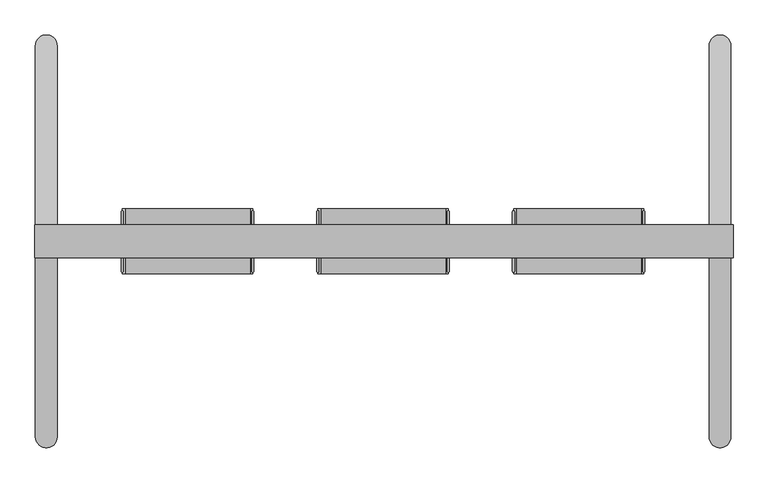
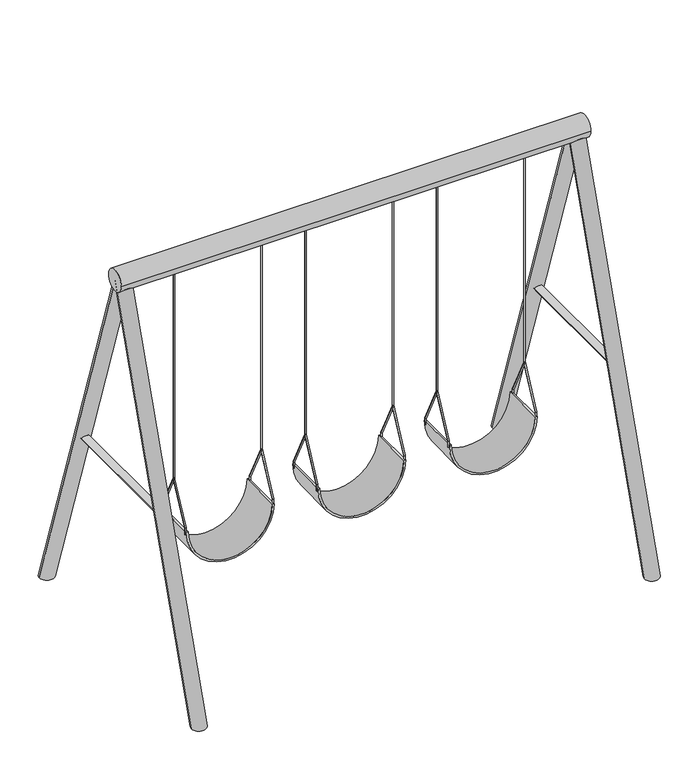
"""IFC4 building model written with IfcOpenShell, lengths in millimetres: geographic element geometry, NLRS_90_SI_WPB_schommel_gen_rsf : schommel drie zittingen."""

from ifc_helpers import new_model, si_unit, point, frame, frame_2d, origin, place, context, project, spatial, polyline, circle_curve, ellipse_curve, trimmed, segment, composite_curve, outline, extrude, source, transform, mapped, element, save
from ifc_brep_helpers import plane_surface, cylinder_surface, extruded_surface, advanced_brep


def geographic_element_11561118(model_context):
    return source(origin(), model_context, "Body", "SolidModel", [
        extrude(outline(composite_curve([segment(trimmed(circle_curve(frame_2d((1554.4555861, -208.1099379)), 4.8239671), [point((1549.631619, -208.1099379))], [point((1559.2795532, -208.1099379))], False, "CARTESIAN"), True, "CONTINUOUS"), segment(trimmed(circle_curve(frame_2d((1554.4555861, -208.1099379)), 4.8239671), [point((1559.2795532, -208.1099379))], [point((1549.631619, -208.1099379))], False, "CARTESIAN"), True, "CONTINUOUS")], self_intersect=False)), frame((0.0, 0.0, 1142.0124483), z_axis=(0.0, 0.0, 1.0), x_axis=(1.0, 0.0, 0.0)), (0.0, 0.0, 1.0), 1601.1875517),
        extrude(outline(composite_curve([segment(trimmed(circle_curve(frame_2d((944.8555861, -208.1099379)), 4.8239671), [point((940.031619, -208.1099379))], [point((949.6795532, -208.1099379))], False, "CARTESIAN"), True, "CONTINUOUS"), segment(trimmed(circle_curve(frame_2d((944.8555861, -208.1099379)), 4.8239671), [point((949.6795532, -208.1099379))], [point((940.031619, -208.1099379))], False, "CARTESIAN"), True, "CONTINUOUS")], self_intersect=False)), frame((0.0, 0.0, 1142.0124483), z_axis=(0.0, 0.0, 1.0), x_axis=(1.0, 0.0, 0.0)), (0.0, 0.0, 1.0), 1601.1875517),
        extrude(outline(composite_curve([segment(trimmed(circle_curve(frame_2d((640.0555861, -208.1099379)), 4.8239671), [point((635.231619, -208.1099379))], [point((644.8795532, -208.1099379))], False, "CARTESIAN"), True, "CONTINUOUS"), segment(trimmed(circle_curve(frame_2d((640.0555861, -208.1099379)), 4.8239671), [point((644.8795532, -208.1099379))], [point((635.231619, -208.1099379))], False, "CARTESIAN"), True, "CONTINUOUS")], self_intersect=False)), frame((0.0, 0.0, 1142.0124483), z_axis=(0.0, 0.0, 1.0), x_axis=(1.0, 0.0, 0.0)), (0.0, 0.0, 1.0), 1601.1875517),
        extrude(outline(composite_curve([segment(trimmed(circle_curve(frame_2d((30.4555861, -208.1099379)), 4.8239671), [point((25.631619, -208.1099379))], [point((35.2795532, -208.1099379))], False, "CARTESIAN"), True, "CONTINUOUS"), segment(trimmed(circle_curve(frame_2d((30.4555861, -208.1099379)), 4.8239671), [point((35.2795532, -208.1099379))], [point((25.631619, -208.1099379))], False, "CARTESIAN"), True, "CONTINUOUS")], self_intersect=False)), frame((0.0, 0.0, 1142.0124483), z_axis=(0.0, 0.0, 1.0), x_axis=(1.0, 0.0, 0.0)), (0.0, 0.0, 1.0), 1601.1875517),
        extrude(outline(composite_curve([segment(trimmed(circle_curve(frame_2d((-274.3444139, -208.1099379)), 4.8239671), [point((-279.168381, -208.1099379))], [point((-269.5204468, -208.1099379))], False, "CARTESIAN"), True, "CONTINUOUS"), segment(trimmed(circle_curve(frame_2d((-274.3444139, -208.1099379)), 4.8239671), [point((-269.5204468, -208.1099379))], [point((-279.168381, -208.1099379))], False, "CARTESIAN"), True, "CONTINUOUS")], self_intersect=False)), frame((0.0, 0.0, 1142.0124483), z_axis=(0.0, 0.0, 1.0), x_axis=(1.0, 0.0, 0.0)), (0.0, 0.0, 1.0), 1601.1875517),
        extrude(outline(composite_curve([segment(trimmed(circle_curve(frame_2d((-884.281587, -208.1099379)), 4.8239671), [point((-889.1055542, -208.1099379))], [point((-879.4576199, -208.1099379))], False, "CARTESIAN"), True, "CONTINUOUS"), segment(trimmed(circle_curve(frame_2d((-884.281587, -208.1099379)), 4.8239671), [point((-879.4576199, -208.1099379))], [point((-889.1055542, -208.1099379))], False, "CARTESIAN"), True, "CONTINUOUS")], self_intersect=False)), frame((0.0, 0.0, 1142.0124483), z_axis=(0.0, 0.0, 1.0), x_axis=(1.0, 0.0, 0.0)), (0.0, 0.0, 1.0), 1601.1875517),
        advanced_brep(
        [(1859.2555861, -1121.8740789, 0.0), (1960.8555861, -1121.8740789, 0.0), (1960.8555861, -207.4740789, 2743.2), (1859.2555861, -207.4740789, 2743.2)],
        [
            (0, 1, circle_curve(frame((1910.0555861, -1121.8740789, 0.0), z_axis=(0.0, 0.0, 1.0), x_axis=(-1.0, 0.0, 0.0)), 50.8)),
            (1, 2),
            (2, 3, circle_curve(frame((1910.0555861, -207.4740789, 2743.2), z_axis=(0.0, 0.0, -1.0), x_axis=(-1.0, 0.0, 0.0)), 50.8)),
            (3, 0),
            (0, 1, circle_curve(frame((1910.0555861, -1121.8740789, 0.0), z_axis=(0.0, 0.0, -1.0), x_axis=(-1.0, 0.0, 0.0)), 50.8)),
            (3, 2, circle_curve(frame((1910.0555861, -207.4740789, 2743.2), z_axis=(0.0, 0.0, -1.0), x_axis=(-1.0, 0.0, 0.0)), 50.8)),
        ],
        [
            extruded_surface(trimmed(circle_curve(frame((1910.0555861, -1121.8740789, 0.0), z_axis=(0.0, 0.0, 1.0), x_axis=(-1.0, 0.0, 0.0)), 50.8), [point((1859.2555861, -1121.8740789, 0.0))], [point((1960.8555861, -1121.8740789, 0.0))], True, "CARTESIAN"), (0.0, 914.4000000000001, 2743.2), 2891.586692457966),
            plane_surface(frame((1910.0555861, -1121.8740789, 0.0), z_axis=(0.0, 0.0, -1.0), x_axis=(0.0, 1.0, 0.0))),
            extruded_surface(trimmed(circle_curve(frame((1910.0555861, -1121.8740789, 0.0), z_axis=(0.0, 0.0, 1.0), x_axis=(-1.0, 0.0, 0.0)), 50.8), [point((1960.8555861, -1121.8740789, 0.0))], [point((1859.2555861, -1121.8740789, 0.0))], True, "CARTESIAN"), (0.0, 914.4000000000001, 2743.2), 2891.586692457966),
            plane_surface(frame((1910.0555861, -207.4740789, 2743.2), z_axis=(0.0, 0.0, 1.0), x_axis=(0.0, 1.0, 0.0))),
        ],
        [
            (0, [[1, 2, 3, 4]]),
            (1, [[-1, 5]]),
            (2, [[-5, -4, 6, -2]]),
            (3, [[-6, -3]]),
        ],
    ),
        advanced_brep(
        [(1859.2555861, 706.9259211, 0.0), (1960.8555861, 706.9259211, 0.0), (1960.8555861, -207.4740789, 2743.2), (1859.2555861, -207.4740789, 2743.2)],
        [
            (0, 1, circle_curve(frame((1910.0555861, 706.9259211, 0.0), z_axis=(0.0, 0.0, 1.0), x_axis=(-1.0, 0.0, 0.0)), 50.8)),
            (1, 2),
            (2, 3, circle_curve(frame((1910.0555861, -207.4740789, 2743.2), z_axis=(0.0, 0.0, -1.0), x_axis=(-1.0, 0.0, 0.0)), 50.8)),
            (3, 0),
            (0, 1, circle_curve(frame((1910.0555861, 706.9259211, 0.0), z_axis=(0.0, 0.0, -1.0), x_axis=(-1.0, 0.0, 0.0)), 50.8)),
            (3, 2, circle_curve(frame((1910.0555861, -207.4740789, 2743.2), z_axis=(0.0, 0.0, -1.0), x_axis=(-1.0, 0.0, 0.0)), 50.8)),
        ],
        [
            extruded_surface(trimmed(circle_curve(frame((1910.0555861, 706.9259211, 0.0), z_axis=(0.0, 0.0, 1.0), x_axis=(-1.0, 0.0, 0.0)), 50.8), [point((1859.2555861, 706.9259211, 0.0))], [point((1960.8555861, 706.9259211, 0.0))], True, "CARTESIAN"), (0.0, -914.4, 2743.2), 2891.586692457966),
            plane_surface(frame((1910.0555861, 706.9259211, 0.0), z_axis=(0.0, 0.0, -1.0), x_axis=(0.0, 1.0, 0.0))),
            extruded_surface(trimmed(circle_curve(frame((1910.0555861, 706.9259211, 0.0), z_axis=(0.0, 0.0, 1.0), x_axis=(-1.0, 0.0, 0.0)), 50.8), [point((1960.8555861, 706.9259211, 0.0))], [point((1859.2555861, 706.9259211, 0.0))], True, "CARTESIAN"), (0.0, -914.4, 2743.2), 2891.586692457966),
            plane_surface(frame((1910.0555861, -207.4740789, 2743.2), z_axis=(0.0, 0.0, 1.0), x_axis=(0.0, 1.0, 0.0))),
        ],
        [
            (0, [[1, 2, 3, 4]]),
            (1, [[-1, 5]]),
            (2, [[-5, -4, 6, -2]]),
            (3, [[-6, -3]]),
        ],
    ),
        advanced_brep(
        [(-1188.7444139, -1121.8740789, 0.0), (-1290.3444139, -1121.8740789, 0.0), (-1290.3444139, -207.4740789, 2743.2), (-1188.7444139, -207.4740789, 2743.2)],
        [
            (0, 1, circle_curve(frame((-1239.5444139, -1121.8740789, 0.0), z_axis=(0.0, 0.0, 1.0), x_axis=(1.0, 0.0, 0.0)), 50.8)),
            (1, 2),
            (2, 3, circle_curve(frame((-1239.5444139, -207.4740789, 2743.2), z_axis=(0.0, 0.0, -1.0), x_axis=(1.0, 0.0, 0.0)), 50.8)),
            (3, 0),
            (0, 1, circle_curve(frame((-1239.5444139, -1121.8740789, 0.0), z_axis=(0.0, 0.0, -1.0), x_axis=(1.0, 0.0, 0.0)), 50.8)),
            (3, 2, circle_curve(frame((-1239.5444139, -207.4740789, 2743.2), z_axis=(0.0, 0.0, -1.0), x_axis=(1.0, 0.0, 0.0)), 50.8)),
        ],
        [
            extruded_surface(trimmed(circle_curve(frame((-1239.5444139, -1121.8740789, 0.0), z_axis=(0.0, 0.0, 1.0), x_axis=(1.0, 0.0, 0.0)), 50.8), [point((-1188.7444139, -1121.8740789, 0.0))], [point((-1290.3444139, -1121.8740789, 0.0))], True, "CARTESIAN"), (0.0, 914.4000000000001, 2743.2), 2891.586692457966),
            plane_surface(frame((-1239.5444139, -1121.8740789, 0.0), z_axis=(0.0, 0.0, -1.0), x_axis=(0.0, -1.0, 0.0))),
            extruded_surface(trimmed(circle_curve(frame((-1239.5444139, -1121.8740789, 0.0), z_axis=(0.0, 0.0, 1.0), x_axis=(1.0, 0.0, 0.0)), 50.8), [point((-1290.3444139, -1121.8740789, 0.0))], [point((-1188.7444139, -1121.8740789, 0.0))], True, "CARTESIAN"), (0.0, 914.4000000000001, 2743.2), 2891.586692457966),
            plane_surface(frame((-1239.5444139, -207.4740789, 2743.2), z_axis=(0.0, 0.0, 1.0), x_axis=(0.0, -1.0, 0.0))),
        ],
        [
            (0, [[1, 2, 3, 4]]),
            (1, [[-1, 5]]),
            (2, [[-5, -4, 6, -2]]),
            (3, [[-6, -3]]),
        ],
    ),
        advanced_brep(
        [(-1188.7444139, 706.9259211, 0.0), (-1290.3444139, 706.9259211, 0.0), (-1290.3444139, -207.4740789, 2743.2), (-1188.7444139, -207.4740789, 2743.2)],
        [
            (0, 1, circle_curve(frame((-1239.5444139, 706.9259211, 0.0), z_axis=(0.0, 0.0, 1.0), x_axis=(1.0, 0.0, 0.0)), 50.8)),
            (1, 2),
            (2, 3, circle_curve(frame((-1239.5444139, -207.4740789, 2743.2), z_axis=(0.0, 0.0, -1.0), x_axis=(1.0, 0.0, 0.0)), 50.8)),
            (3, 0),
            (0, 1, circle_curve(frame((-1239.5444139, 706.9259211, 0.0), z_axis=(0.0, 0.0, -1.0), x_axis=(1.0, 0.0, 0.0)), 50.8)),
            (3, 2, circle_curve(frame((-1239.5444139, -207.4740789, 2743.2), z_axis=(0.0, 0.0, -1.0), x_axis=(1.0, 0.0, 0.0)), 50.8)),
        ],
        [
            extruded_surface(trimmed(circle_curve(frame((-1239.5444139, 706.9259211, 0.0), z_axis=(0.0, 0.0, 1.0), x_axis=(1.0, 0.0, 0.0)), 50.8), [point((-1188.7444139, 706.9259211, 0.0))], [point((-1290.3444139, 706.9259211, 0.0))], True, "CARTESIAN"), (0.0, -914.4, 2743.2), 2891.586692457966),
            plane_surface(frame((-1239.5444139, 706.9259211, 0.0), z_axis=(0.0, 0.0, -1.0), x_axis=(0.0, -1.0, 0.0))),
            extruded_surface(trimmed(circle_curve(frame((-1239.5444139, 706.9259211, 0.0), z_axis=(0.0, 0.0, 1.0), x_axis=(1.0, 0.0, 0.0)), 50.8), [point((-1290.3444139, 706.9259211, 0.0))], [point((-1188.7444139, 706.9259211, 0.0))], True, "CARTESIAN"), (0.0, -914.4, 2743.2), 2891.586692457966),
            plane_surface(frame((-1239.5444139, -207.4740789, 2743.2), z_axis=(0.0, 0.0, 1.0), x_axis=(0.0, -1.0, 0.0))),
        ],
        [
            (0, [[1, 2, 3, 4]]),
            (1, [[-1, 5]]),
            (2, [[-5, -4, 6, -2]]),
            (3, [[-6, -3]]),
        ],
    ),
        extrude(outline(composite_curve([segment(trimmed(circle_curve(frame_2d((-207.4740789, 2743.2)), 76.2), [point((-131.2740789, 2743.2))], [point((-283.6740789, 2743.2))], False, "CARTESIAN"), True, "CONTINUOUS"), segment(trimmed(circle_curve(frame_2d((-207.4740789, 2743.2)), 76.2), [point((-283.6740789, 2743.2))], [point((-131.2740789, 2743.2))], False, "CARTESIAN"), True, "CONTINUOUS")], self_intersect=False)), frame((-1292.7850188, 0.0, 0.0), z_axis=(1.0, 0.0, 0.0), x_axis=(0.0, 1.0, 0.0)), (0.0, 0.0, 1.0), 3264.3036372),
        advanced_brep(
        [(1549.631619, -69.3189818, 818.7879391), (1559.2795532, -69.3189818, 818.7879391), (1549.631619, -69.3189818, 863.2379391), (1559.2795532, -69.3189818, 863.2379391), (1549.631619, -208.1099379, 1142.0124483), (1559.2795532, -208.1099379, 1142.0124483), (1549.631619, -346.9008939, 863.2379391), (1559.2795532, -346.9008939, 863.2379391), (1549.631619, -346.9008939, 818.7879391), (1559.2795532, -346.9008939, 818.7879391)],
        [
            (0, 1, circle_curve(frame((1554.4555861, -69.3189818, 818.7879391), z_axis=(0.0, 0.0, -1.0), x_axis=(1.0, 0.0, 0.0)), 4.8239671)),
            (1, 0, circle_curve(frame((1554.4555861, -69.3189818, 818.7879391), z_axis=(0.0, 0.0, -1.0), x_axis=(1.0, 0.0, 0.0)), 4.8239671)),
            (0, 2),
            (2, 3, ellipse_curve(frame((1554.4555861, -69.3189818, 863.2379391), z_axis=(0.0, 0.22891941247129147, -0.9734453773036259), x_axis=(0.0, -0.973445377303626, -0.22891941247129194)), 4.9555602, 4.8239671)),
            (3, 1),
            (3, 2, ellipse_curve(frame((1554.4555861, -69.3189818, 863.2379391), z_axis=(0.0, 0.22891941247129147, -0.9734453773036259), x_axis=(0.0, -0.973445377303626, -0.22891941247129194)), 4.9555602, 4.8239671)),
            (2, 4),
            (4, 5, ellipse_curve(frame((1554.4555861, -208.1099379, 1142.0124483), z_axis=(0.0, 1.0, 0.0), x_axis=(0.0, 0.0, -1.0)), 10.8238094, 4.8239671)),
            (5, 3),
            (5, 4, ellipse_curve(frame((1554.4555861, -208.1099379, 1142.0124483), z_axis=(0.0, 1.0, 0.0), x_axis=(0.0, 0.0, -1.0)), 10.8238094, 4.8239671)),
            (4, 6),
            (6, 7, ellipse_curve(frame((1554.4555861, -346.9008939, 863.2379391), z_axis=(0.0, 0.22891941247129094, 0.973445377303626), x_axis=(0.0, 0.9734453773036262, -0.22891941247129044)), 4.9555602, 4.8239671)),
            (7, 5),
            (7, 6, ellipse_curve(frame((1554.4555861, -346.9008939, 863.2379391), z_axis=(0.0, 0.22891941247129094, 0.973445377303626), x_axis=(0.0, 0.9734453773036262, -0.22891941247129044)), 4.9555602, 4.8239671)),
            (8, 9, circle_curve(frame((1554.4555861, -346.9008939, 818.7879391), z_axis=(0.0, 0.0, -1.0), x_axis=(1.0, 0.0, 0.0)), 4.8239671)),
            (9, 8, circle_curve(frame((1554.4555861, -346.9008939, 818.7879391), z_axis=(0.0, 0.0, -1.0), x_axis=(1.0, 0.0, 0.0)), 4.8239671)),
            (6, 8),
            (9, 7),
        ],
        [
            plane_surface(frame((1554.4555861, -69.3189818, 818.7879391), z_axis=(0.0, 0.0, -1.0), x_axis=(-1.0, 0.0, 0.0))),
            cylinder_surface(frame((1554.4555861, -69.3189818, 818.7879391), z_axis=(0.0, 0.0, -1.0), x_axis=(1.0, 0.0, 0.0)), 4.8239671),
            cylinder_surface(frame((1554.4555861, -69.3189818, 863.2379391), z_axis=(0.0, 0.44568108769047987, -0.8951918051875982), x_axis=(1.0, 0.0, 0.0)), 4.8239671),
            cylinder_surface(frame((1554.4555861, -208.1099379, 1142.0124483), z_axis=(0.0, 0.4456810876904795, 0.8951918051875986), x_axis=(1.0, 0.0, 0.0)), 4.8239671),
            plane_surface(frame((1554.4555861, -346.9008939, 818.7879391), z_axis=(0.0, 0.0, -1.0), x_axis=(-1.0, 0.0, 0.0))),
            cylinder_surface(frame((1554.4555861, -346.9008939, 863.2379391), z_axis=(0.0, 0.0, 1.0), x_axis=(1.0, 0.0, 0.0)), 4.8239671),
        ],
        [
            (0, [[1, 2]]),
            (1, [[-1, 3, 4, 5]]),
            (1, [[-2, -5, 6, -3]]),
            (2, [[-4, 7, 8, 9]]),
            (2, [[-6, -9, 10, -7]]),
            (3, [[-8, 11, 12, 13]]),
            (3, [[-10, -13, 14, -11]]),
            (4, [[15, 16]]),
            (5, [[-12, 17, -16, 18]]),
            (5, [[-14, -18, -15, -17]]),
        ],
    ),
        advanced_brep(
        [(940.031619, -69.3189818, 818.7879391), (949.6795532, -69.3189818, 818.7879391), (940.031619, -69.3189818, 863.2379391), (949.6795532, -69.3189818, 863.2379391), (940.031619, -208.1099379, 1142.0124483), (949.6795532, -208.1099379, 1142.0124483), (940.031619, -346.9008939, 863.2379391), (949.6795532, -346.9008939, 863.2379391), (940.031619, -346.9008939, 818.7879391), (949.6795532, -346.9008939, 818.7879391)],
        [
            (0, 1, circle_curve(frame((944.8555861, -69.3189818, 818.7879391), z_axis=(0.0, 0.0, -1.0), x_axis=(1.0, 0.0, 0.0)), 4.8239671)),
            (1, 0, circle_curve(frame((944.8555861, -69.3189818, 818.7879391), z_axis=(0.0, 0.0, -1.0), x_axis=(1.0, 0.0, 0.0)), 4.8239671)),
            (0, 2),
            (2, 3, ellipse_curve(frame((944.8555861, -69.3189818, 863.2379391), z_axis=(0.0, 0.22891941247129147, -0.9734453773036259), x_axis=(0.0, -0.973445377303626, -0.22891941247129194)), 4.9555602, 4.8239671)),
            (3, 1),
            (3, 2, ellipse_curve(frame((944.8555861, -69.3189818, 863.2379391), z_axis=(0.0, 0.22891941247129147, -0.9734453773036259), x_axis=(0.0, -0.973445377303626, -0.22891941247129194)), 4.9555602, 4.8239671)),
            (2, 4),
            (4, 5, ellipse_curve(frame((944.8555861, -208.1099379, 1142.0124483), z_axis=(0.0, 1.0, 0.0), x_axis=(0.0, 0.0, -1.0)), 10.8238094, 4.8239671)),
            (5, 3),
            (5, 4, ellipse_curve(frame((944.8555861, -208.1099379, 1142.0124483), z_axis=(0.0, 1.0, 0.0), x_axis=(0.0, 0.0, -1.0)), 10.8238094, 4.8239671)),
            (4, 6),
            (6, 7, ellipse_curve(frame((944.8555861, -346.9008939, 863.2379391), z_axis=(0.0, 0.22891941247129094, 0.973445377303626), x_axis=(0.0, 0.9734453773036262, -0.22891941247129044)), 4.9555602, 4.8239671)),
            (7, 5),
            (7, 6, ellipse_curve(frame((944.8555861, -346.9008939, 863.2379391), z_axis=(0.0, 0.22891941247129094, 0.973445377303626), x_axis=(0.0, 0.9734453773036262, -0.22891941247129044)), 4.9555602, 4.8239671)),
            (8, 9, circle_curve(frame((944.8555861, -346.9008939, 818.7879391), z_axis=(0.0, 0.0, -1.0), x_axis=(1.0, 0.0, 0.0)), 4.8239671)),
            (9, 8, circle_curve(frame((944.8555861, -346.9008939, 818.7879391), z_axis=(0.0, 0.0, -1.0), x_axis=(1.0, 0.0, 0.0)), 4.8239671)),
            (6, 8),
            (9, 7),
        ],
        [
            plane_surface(frame((944.8555861, -69.3189818, 818.7879391), z_axis=(0.0, 0.0, -1.0), x_axis=(-1.0, 0.0, 0.0))),
            cylinder_surface(frame((944.8555861, -69.3189818, 818.7879391), z_axis=(0.0, 0.0, -1.0), x_axis=(1.0, 0.0, 0.0)), 4.8239671),
            cylinder_surface(frame((944.8555861, -69.3189818, 863.2379391), z_axis=(0.0, 0.44568108769047987, -0.8951918051875982), x_axis=(1.0, 0.0, 0.0)), 4.8239671),
            cylinder_surface(frame((944.8555861, -208.1099379, 1142.0124483), z_axis=(0.0, 0.4456810876904795, 0.8951918051875986), x_axis=(1.0, 0.0, 0.0)), 4.8239671),
            plane_surface(frame((944.8555861, -346.9008939, 818.7879391), z_axis=(0.0, 0.0, -1.0), x_axis=(-1.0, 0.0, 0.0))),
            cylinder_surface(frame((944.8555861, -346.9008939, 863.2379391), z_axis=(0.0, 0.0, 1.0), x_axis=(1.0, 0.0, 0.0)), 4.8239671),
        ],
        [
            (0, [[1, 2]]),
            (1, [[-1, 3, 4, 5]]),
            (1, [[-2, -5, 6, -3]]),
            (2, [[-4, 7, 8, 9]]),
            (2, [[-6, -9, 10, -7]]),
            (3, [[-8, 11, 12, 13]]),
            (3, [[-10, -13, 14, -11]]),
            (4, [[15, 16]]),
            (5, [[-12, 17, -16, 18]]),
            (5, [[-14, -18, -15, -17]]),
        ],
    ),
        advanced_brep(
        [(635.231619, -69.3189818, 818.7879391), (644.8795532, -69.3189818, 818.7879391), (635.231619, -69.3189818, 863.2379391), (644.8795532, -69.3189818, 863.2379391), (635.231619, -208.1099379, 1142.0124483), (644.8795532, -208.1099379, 1142.0124483), (635.231619, -346.9008939, 863.2379391), (644.8795532, -346.9008939, 863.2379391), (635.231619, -346.9008939, 818.7879391), (644.8795532, -346.9008939, 818.7879391)],
        [
            (0, 1, circle_curve(frame((640.0555861, -69.3189818, 818.7879391), z_axis=(0.0, 0.0, -1.0), x_axis=(1.0, 0.0, 0.0)), 4.8239671)),
            (1, 0, circle_curve(frame((640.0555861, -69.3189818, 818.7879391), z_axis=(0.0, 0.0, -1.0), x_axis=(1.0, 0.0, 0.0)), 4.8239671)),
            (0, 2),
            (2, 3, ellipse_curve(frame((640.0555861, -69.3189818, 863.2379391), z_axis=(0.0, 0.22891941247129147, -0.9734453773036259), x_axis=(0.0, -0.973445377303626, -0.22891941247129194)), 4.9555602, 4.8239671)),
            (3, 1),
            (3, 2, ellipse_curve(frame((640.0555861, -69.3189818, 863.2379391), z_axis=(0.0, 0.22891941247129147, -0.9734453773036259), x_axis=(0.0, -0.973445377303626, -0.22891941247129194)), 4.9555602, 4.8239671)),
            (2, 4),
            (4, 5, ellipse_curve(frame((640.0555861, -208.1099379, 1142.0124483), z_axis=(0.0, 1.0, 0.0), x_axis=(0.0, 0.0, -1.0)), 10.8238094, 4.8239671)),
            (5, 3),
            (5, 4, ellipse_curve(frame((640.0555861, -208.1099379, 1142.0124483), z_axis=(0.0, 1.0, 0.0), x_axis=(0.0, 0.0, -1.0)), 10.8238094, 4.8239671)),
            (4, 6),
            (6, 7, ellipse_curve(frame((640.0555861, -346.9008939, 863.2379391), z_axis=(0.0, 0.22891941247129094, 0.973445377303626), x_axis=(0.0, 0.9734453773036262, -0.22891941247129044)), 4.9555602, 4.8239671)),
            (7, 5),
            (7, 6, ellipse_curve(frame((640.0555861, -346.9008939, 863.2379391), z_axis=(0.0, 0.22891941247129094, 0.973445377303626), x_axis=(0.0, 0.9734453773036262, -0.22891941247129044)), 4.9555602, 4.8239671)),
            (8, 9, circle_curve(frame((640.0555861, -346.9008939, 818.7879391), z_axis=(0.0, 0.0, -1.0), x_axis=(1.0, 0.0, 0.0)), 4.8239671)),
            (9, 8, circle_curve(frame((640.0555861, -346.9008939, 818.7879391), z_axis=(0.0, 0.0, -1.0), x_axis=(1.0, 0.0, 0.0)), 4.8239671)),
            (6, 8),
            (9, 7),
        ],
        [
            plane_surface(frame((640.0555861, -69.3189818, 818.7879391), z_axis=(0.0, 0.0, -1.0), x_axis=(-1.0, 0.0, 0.0))),
            cylinder_surface(frame((640.0555861, -69.3189818, 818.7879391), z_axis=(0.0, 0.0, -1.0), x_axis=(1.0, 0.0, 0.0)), 4.8239671),
            cylinder_surface(frame((640.0555861, -69.3189818, 863.2379391), z_axis=(0.0, 0.44568108769047987, -0.8951918051875982), x_axis=(1.0, 0.0, 0.0)), 4.8239671),
            cylinder_surface(frame((640.0555861, -208.1099379, 1142.0124483), z_axis=(0.0, 0.4456810876904795, 0.8951918051875986), x_axis=(1.0, 0.0, 0.0)), 4.8239671),
            plane_surface(frame((640.0555861, -346.9008939, 818.7879391), z_axis=(0.0, 0.0, -1.0), x_axis=(-1.0, 0.0, 0.0))),
            cylinder_surface(frame((640.0555861, -346.9008939, 863.2379391), z_axis=(0.0, 0.0, 1.0), x_axis=(1.0, 0.0, 0.0)), 4.8239671),
        ],
        [
            (0, [[1, 2]]),
            (1, [[-1, 3, 4, 5]]),
            (1, [[-2, -5, 6, -3]]),
            (2, [[-4, 7, 8, 9]]),
            (2, [[-6, -9, 10, -7]]),
            (3, [[-8, 11, 12, 13]]),
            (3, [[-10, -13, 14, -11]]),
            (4, [[15, 16]]),
            (5, [[-12, 17, -16, 18]]),
            (5, [[-14, -18, -15, -17]]),
        ],
    ),
        advanced_brep(
        [(25.631619, -69.3189818, 818.7879391), (35.2795532, -69.3189818, 818.7879391), (25.631619, -69.3189818, 863.2379391), (35.2795532, -69.3189818, 863.2379391), (25.631619, -208.1099379, 1142.0124483), (35.2795532, -208.1099379, 1142.0124483), (25.631619, -346.9008939, 863.2379391), (35.2795532, -346.9008939, 863.2379391), (25.631619, -346.9008939, 818.7879391), (35.2795532, -346.9008939, 818.7879391)],
        [
            (0, 1, circle_curve(frame((30.4555861, -69.3189818, 818.7879391), z_axis=(0.0, 0.0, -1.0), x_axis=(1.0, 0.0, 0.0)), 4.8239671)),
            (1, 0, circle_curve(frame((30.4555861, -69.3189818, 818.7879391), z_axis=(0.0, 0.0, -1.0), x_axis=(1.0, 0.0, 0.0)), 4.8239671)),
            (0, 2),
            (2, 3, ellipse_curve(frame((30.4555861, -69.3189818, 863.2379391), z_axis=(0.0, 0.22891941247129147, -0.9734453773036259), x_axis=(0.0, -0.973445377303626, -0.22891941247129194)), 4.9555602, 4.8239671)),
            (3, 1),
            (3, 2, ellipse_curve(frame((30.4555861, -69.3189818, 863.2379391), z_axis=(0.0, 0.22891941247129147, -0.9734453773036259), x_axis=(0.0, -0.973445377303626, -0.22891941247129194)), 4.9555602, 4.8239671)),
            (2, 4),
            (4, 5, ellipse_curve(frame((30.4555861, -208.1099379, 1142.0124483), z_axis=(0.0, 1.0, 0.0), x_axis=(0.0, 0.0, -1.0)), 10.8238094, 4.8239671)),
            (5, 3),
            (5, 4, ellipse_curve(frame((30.4555861, -208.1099379, 1142.0124483), z_axis=(0.0, 1.0, 0.0), x_axis=(0.0, 0.0, -1.0)), 10.8238094, 4.8239671)),
            (4, 6),
            (6, 7, ellipse_curve(frame((30.4555861, -346.9008939, 863.2379391), z_axis=(0.0, 0.22891941247129094, 0.973445377303626), x_axis=(0.0, 0.9734453773036262, -0.22891941247129044)), 4.9555602, 4.8239671)),
            (7, 5),
            (7, 6, ellipse_curve(frame((30.4555861, -346.9008939, 863.2379391), z_axis=(0.0, 0.22891941247129094, 0.973445377303626), x_axis=(0.0, 0.9734453773036262, -0.22891941247129044)), 4.9555602, 4.8239671)),
            (8, 9, circle_curve(frame((30.4555861, -346.9008939, 818.7879391), z_axis=(0.0, 0.0, -1.0), x_axis=(1.0, 0.0, 0.0)), 4.8239671)),
            (9, 8, circle_curve(frame((30.4555861, -346.9008939, 818.7879391), z_axis=(0.0, 0.0, -1.0), x_axis=(1.0, 0.0, 0.0)), 4.8239671)),
            (6, 8),
            (9, 7),
        ],
        [
            plane_surface(frame((30.4555861, -69.3189818, 818.7879391), z_axis=(0.0, 0.0, -1.0), x_axis=(-1.0, 0.0, 0.0))),
            cylinder_surface(frame((30.4555861, -69.3189818, 818.7879391), z_axis=(0.0, 0.0, -1.0), x_axis=(1.0, 0.0, 0.0)), 4.8239671),
            cylinder_surface(frame((30.4555861, -69.3189818, 863.2379391), z_axis=(0.0, 0.44568108769047987, -0.8951918051875982), x_axis=(1.0, 0.0, 0.0)), 4.8239671),
            cylinder_surface(frame((30.4555861, -208.1099379, 1142.0124483), z_axis=(0.0, 0.4456810876904795, 0.8951918051875986), x_axis=(1.0, 0.0, 0.0)), 4.8239671),
            plane_surface(frame((30.4555861, -346.9008939, 818.7879391), z_axis=(0.0, 0.0, -1.0), x_axis=(-1.0, 0.0, 0.0))),
            cylinder_surface(frame((30.4555861, -346.9008939, 863.2379391), z_axis=(0.0, 0.0, 1.0), x_axis=(1.0, 0.0, 0.0)), 4.8239671),
        ],
        [
            (0, [[1, 2]]),
            (1, [[-1, 3, 4, 5]]),
            (1, [[-2, -5, 6, -3]]),
            (2, [[-4, 7, 8, 9]]),
            (2, [[-6, -9, 10, -7]]),
            (3, [[-8, 11, 12, 13]]),
            (3, [[-10, -13, 14, -11]]),
            (4, [[15, 16]]),
            (5, [[-12, 17, -16, 18]]),
            (5, [[-14, -18, -15, -17]]),
        ],
    ),
        advanced_brep(
        [(-279.168381, -69.3189818, 818.7879391), (-269.5204468, -69.3189818, 818.7879391), (-279.168381, -69.3189818, 863.2379391), (-269.5204468, -69.3189818, 863.2379391), (-279.168381, -208.1099379, 1142.0124483), (-269.5204468, -208.1099379, 1142.0124483), (-279.168381, -346.9008939, 863.2379391), (-269.5204468, -346.9008939, 863.2379391), (-279.168381, -346.9008939, 818.7879391), (-269.5204468, -346.9008939, 818.7879391)],
        [
            (0, 1, circle_curve(frame((-274.3444139, -69.3189818, 818.7879391), z_axis=(0.0, 0.0, -1.0), x_axis=(1.0, 0.0, 0.0)), 4.8239671)),
            (1, 0, circle_curve(frame((-274.3444139, -69.3189818, 818.7879391), z_axis=(0.0, 0.0, -1.0), x_axis=(1.0, 0.0, 0.0)), 4.8239671)),
            (0, 2),
            (2, 3, ellipse_curve(frame((-274.3444139, -69.3189818, 863.2379391), z_axis=(0.0, 0.22891941247129147, -0.9734453773036259), x_axis=(0.0, -0.973445377303626, -0.22891941247129194)), 4.9555602, 4.8239671)),
            (3, 1),
            (3, 2, ellipse_curve(frame((-274.3444139, -69.3189818, 863.2379391), z_axis=(0.0, 0.22891941247129147, -0.9734453773036259), x_axis=(0.0, -0.973445377303626, -0.22891941247129194)), 4.9555602, 4.8239671)),
            (2, 4),
            (4, 5, ellipse_curve(frame((-274.3444139, -208.1099379, 1142.0124483), z_axis=(0.0, 1.0, 0.0), x_axis=(0.0, 0.0, -1.0)), 10.8238094, 4.8239671)),
            (5, 3),
            (5, 4, ellipse_curve(frame((-274.3444139, -208.1099379, 1142.0124483), z_axis=(0.0, 1.0, 0.0), x_axis=(0.0, 0.0, -1.0)), 10.8238094, 4.8239671)),
            (4, 6),
            (6, 7, ellipse_curve(frame((-274.3444139, -346.9008939, 863.2379391), z_axis=(0.0, 0.22891941247129094, 0.973445377303626), x_axis=(0.0, 0.9734453773036262, -0.22891941247129044)), 4.9555602, 4.8239671)),
            (7, 5),
            (7, 6, ellipse_curve(frame((-274.3444139, -346.9008939, 863.2379391), z_axis=(0.0, 0.22891941247129094, 0.973445377303626), x_axis=(0.0, 0.9734453773036262, -0.22891941247129044)), 4.9555602, 4.8239671)),
            (8, 9, circle_curve(frame((-274.3444139, -346.9008939, 818.7879391), z_axis=(0.0, 0.0, -1.0), x_axis=(1.0, 0.0, 0.0)), 4.8239671)),
            (9, 8, circle_curve(frame((-274.3444139, -346.9008939, 818.7879391), z_axis=(0.0, 0.0, -1.0), x_axis=(1.0, 0.0, 0.0)), 4.8239671)),
            (6, 8),
            (9, 7),
        ],
        [
            plane_surface(frame((-274.3444139, -69.3189818, 818.7879391), z_axis=(0.0, 0.0, -1.0), x_axis=(-1.0, 0.0, 0.0))),
            cylinder_surface(frame((-274.3444139, -69.3189818, 818.7879391), z_axis=(0.0, 0.0, -1.0), x_axis=(1.0, 0.0, 0.0)), 4.8239671),
            cylinder_surface(frame((-274.3444139, -69.3189818, 863.2379391), z_axis=(0.0, 0.44568108769047987, -0.8951918051875982), x_axis=(1.0, 0.0, 0.0)), 4.8239671),
            cylinder_surface(frame((-274.3444139, -208.1099379, 1142.0124483), z_axis=(0.0, 0.4456810876904795, 0.8951918051875986), x_axis=(1.0, 0.0, 0.0)), 4.8239671),
            plane_surface(frame((-274.3444139, -346.9008939, 818.7879391), z_axis=(0.0, 0.0, -1.0), x_axis=(-1.0, 0.0, 0.0))),
            cylinder_surface(frame((-274.3444139, -346.9008939, 863.2379391), z_axis=(0.0, 0.0, 1.0), x_axis=(1.0, 0.0, 0.0)), 4.8239671),
        ],
        [
            (0, [[1, 2]]),
            (1, [[-1, 3, 4, 5]]),
            (1, [[-2, -5, 6, -3]]),
            (2, [[-4, 7, 8, 9]]),
            (2, [[-6, -9, 10, -7]]),
            (3, [[-8, 11, 12, 13]]),
            (3, [[-10, -13, 14, -11]]),
            (4, [[15, 16]]),
            (5, [[-12, 17, -16, 18]]),
            (5, [[-14, -18, -15, -17]]),
        ],
    ),
        advanced_brep(
        [(-889.1055542, -69.3189818, 818.7879391), (-879.4576199, -69.3189818, 818.7879391), (-889.1055542, -69.3189818, 863.2379391), (-879.4576199, -69.3189818, 863.2379391), (-889.1055542, -208.1099379, 1142.0124483), (-879.4576199, -208.1099379, 1142.0124483), (-889.1055542, -346.9008939, 863.2379391), (-879.4576199, -346.9008939, 863.2379391), (-889.1055542, -346.9008939, 818.7879391), (-879.4576199, -346.9008939, 818.7879391)],
        [
            (0, 1, circle_curve(frame((-884.281587, -69.3189818, 818.7879391), z_axis=(0.0, 0.0, -1.0), x_axis=(1.0, 0.0, 0.0)), 4.8239671)),
            (1, 0, circle_curve(frame((-884.281587, -69.3189818, 818.7879391), z_axis=(0.0, 0.0, -1.0), x_axis=(1.0, 0.0, 0.0)), 4.8239671)),
            (0, 2),
            (2, 3, ellipse_curve(frame((-884.281587, -69.3189818, 863.2379391), z_axis=(0.0, 0.22891941247129147, -0.9734453773036259), x_axis=(0.0, -0.973445377303626, -0.22891941247129194)), 4.9555602, 4.8239671)),
            (3, 1),
            (3, 2, ellipse_curve(frame((-884.281587, -69.3189818, 863.2379391), z_axis=(0.0, 0.22891941247129147, -0.9734453773036259), x_axis=(0.0, -0.973445377303626, -0.22891941247129194)), 4.9555602, 4.8239671)),
            (2, 4),
            (4, 5, ellipse_curve(frame((-884.281587, -208.1099379, 1142.0124483), z_axis=(0.0, 1.0, 0.0), x_axis=(0.0, 0.0, -1.0)), 10.8238094, 4.8239671)),
            (5, 3),
            (5, 4, ellipse_curve(frame((-884.281587, -208.1099379, 1142.0124483), z_axis=(0.0, 1.0, 0.0), x_axis=(0.0, 0.0, -1.0)), 10.8238094, 4.8239671)),
            (4, 6),
            (6, 7, ellipse_curve(frame((-884.281587, -346.9008939, 863.2379391), z_axis=(0.0, 0.22891941247129094, 0.973445377303626), x_axis=(0.0, 0.9734453773036262, -0.22891941247129044)), 4.9555602, 4.8239671)),
            (7, 5),
            (7, 6, ellipse_curve(frame((-884.281587, -346.9008939, 863.2379391), z_axis=(0.0, 0.22891941247129094, 0.973445377303626), x_axis=(0.0, 0.9734453773036262, -0.22891941247129044)), 4.9555602, 4.8239671)),
            (8, 9, circle_curve(frame((-884.281587, -346.9008939, 818.7879391), z_axis=(0.0, 0.0, -1.0), x_axis=(1.0, 0.0, 0.0)), 4.8239671)),
            (9, 8, circle_curve(frame((-884.281587, -346.9008939, 818.7879391), z_axis=(0.0, 0.0, -1.0), x_axis=(1.0, 0.0, 0.0)), 4.8239671)),
            (6, 8),
            (9, 7),
        ],
        [
            plane_surface(frame((-884.281587, -69.3189818, 818.7879391), z_axis=(0.0, 0.0, -1.0), x_axis=(-1.0, 0.0, 0.0))),
            cylinder_surface(frame((-884.281587, -69.3189818, 818.7879391), z_axis=(0.0, 0.0, -1.0), x_axis=(1.0, 0.0, 0.0)), 4.8239671),
            cylinder_surface(frame((-884.281587, -69.3189818, 863.2379391), z_axis=(0.0, 0.44568108769047987, -0.8951918051875982), x_axis=(1.0, 0.0, 0.0)), 4.8239671),
            cylinder_surface(frame((-884.281587, -208.1099379, 1142.0124483), z_axis=(0.0, 0.4456810876904795, 0.8951918051875986), x_axis=(1.0, 0.0, 0.0)), 4.8239671),
            plane_surface(frame((-884.281587, -346.9008939, 818.7879391), z_axis=(0.0, 0.0, -1.0), x_axis=(-1.0, 0.0, 0.0))),
            cylinder_surface(frame((-884.281587, -346.9008939, 863.2379391), z_axis=(0.0, 0.0, 1.0), x_axis=(1.0, 0.0, 0.0)), 4.8239671),
        ],
        [
            (0, [[1, 2]]),
            (1, [[-1, 3, 4, 5]]),
            (1, [[-2, -5, 6, -3]]),
            (2, [[-4, 7, 8, 9]]),
            (2, [[-6, -9, 10, -7]]),
            (3, [[-8, 11, 12, 13]]),
            (3, [[-10, -13, 14, -11]]),
            (4, [[15, 16]]),
            (5, [[-12, 17, -16, 18]]),
            (5, [[-14, -18, -15, -17]]),
        ],
    ),
        extrude(outline(composite_curve([segment(trimmed(circle_curve(frame_2d((838.2, 1249.6555861)), 292.1), [point((838.2, 1541.7555861))], [point((838.2, 957.5555861))], True, "CARTESIAN"), True, "CONTINUOUS"), segment(polyline([(838.2, 957.5555861), (838.2, 944.8555861)]), True, "CONTINUOUS"), segment(trimmed(circle_curve(frame_2d((838.2, 1249.6555861)), 304.8), [point((838.2, 944.8555861))], [point((838.2, 1554.4555861))], False, "CARTESIAN"), True, "CONTINUOUS"), segment(polyline([(838.2, 1554.4555861), (838.2, 1541.7555861)]), True, "CONTINUOUS")], self_intersect=False)), frame((0.0, -359.8740789, 0.0), z_axis=(0.0, 1.0, 0.0), x_axis=(0.0, 0.0, 1.0)), (0.0, 0.0, 1.0), 304.8),
        extrude(outline(composite_curve([segment(trimmed(circle_curve(frame_2d((838.2, 335.2555861)), 292.1), [point((838.2, 627.3555861))], [point((838.2, 43.1555861))], True, "CARTESIAN"), True, "CONTINUOUS"), segment(polyline([(838.2, 43.1555861), (838.2, 30.4555861)]), True, "CONTINUOUS"), segment(trimmed(circle_curve(frame_2d((838.2, 335.2555861)), 304.8), [point((838.2, 30.4555861))], [point((838.2, 640.0555861))], False, "CARTESIAN"), True, "CONTINUOUS"), segment(polyline([(838.2, 640.0555861), (838.2, 627.3555861)]), True, "CONTINUOUS")], self_intersect=False)), frame((0.0, -359.8740789, 0.0), z_axis=(0.0, 1.0, 0.0), x_axis=(0.0, 0.0, 1.0)), (0.0, 0.0, 1.0), 304.8),
        extrude(outline(composite_curve([segment(trimmed(circle_curve(frame_2d((838.2, -579.1444139)), 292.1), [point((838.2, -287.0444139))], [point((838.2, -871.2444139))], True, "CARTESIAN"), True, "CONTINUOUS"), segment(polyline([(838.2, -871.2444139), (838.2, -883.9444139)]), True, "CONTINUOUS"), segment(trimmed(circle_curve(frame_2d((838.2, -579.1444139)), 304.8), [point((838.2, -883.9444139))], [point((838.2, -274.3444139))], False, "CARTESIAN"), True, "CONTINUOUS"), segment(polyline([(838.2, -274.3444139), (838.2, -287.0444139)]), True, "CONTINUOUS")], self_intersect=False)), frame((0.0, -359.8740789, 0.0), z_axis=(0.0, 1.0, 0.0), x_axis=(0.0, 0.0, 1.0)), (0.0, 0.0, 1.0), 304.8),
        extrude(outline(composite_curve([segment(trimmed(circle_curve(frame_2d((1306.4836451, -1245.8756596)), 25.4), [point((1306.4836451, -1271.2756596))], [point((1306.4836451, -1220.4756596))], False, "CARTESIAN"), True, "CONTINUOUS"), segment(trimmed(circle_curve(frame_2d((1306.4836451, -1245.8756596)), 25.4), [point((1306.4836451, -1220.4756596))], [point((1306.4836451, -1271.2756596))], False, "CARTESIAN"), True, "CONTINUOUS")], self_intersect=False)), frame((0.0, -677.6736483, 0.0), z_axis=(0.0, 1.0, 0.0), x_axis=(0.0, 0.0, 1.0)), (0.0, 0.0, 1.0), 943.7306176),
        extrude(outline(composite_curve([segment(trimmed(circle_curve(frame_2d((1306.4836451, 1903.6868318)), 25.4), [point((1306.4836451, 1929.0868318))], [point((1306.4836451, 1878.2868318))], False, "CARTESIAN"), True, "CONTINUOUS"), segment(trimmed(circle_curve(frame_2d((1306.4836451, 1903.6868318)), 25.4), [point((1306.4836451, 1878.2868318))], [point((1306.4836451, 1929.0868318))], False, "CARTESIAN"), True, "CONTINUOUS")], self_intersect=False)), frame((0.0, -677.6736483, 0.0), z_axis=(0.0, 1.0, 0.0), x_axis=(0.0, 0.0, 1.0)), (0.0, 0.0, 1.0), 943.7306176),
    ])


if __name__ == "__main__":
    model = new_model("IFC4")
    model_context = context("Model", 3, world=origin())
    ifc_project = project(units=[si_unit("LENGTHUNIT", "METRE", prefix="MILLI")], contexts=[model_context])
    site = spatial("IfcSite", under=ifc_project)
    building = spatial("IfcBuilding", under=site)
    placement = place(None, origin())
    geographic_element_shape = geographic_element_11561118(model_context)
    element("IfcGeographicElement", 1, ObjectType="NLRS_90_SI_WPB_schommel_gen_rsf : schommel drie zittingen", at=placement, inside=building, context=model_context, shape_type="MappedRepresentation", body=[
        mapped(geographic_element_shape, transform((0.0, 0.0, 0.0), x_axis=(1.0, 0.0, 0.0), y_axis=(0.0, 1.0, 0.0), z_axis=(0.0, 0.0, 1.0))),
    ])
    save(model, "model.ifc")

# Revit data of these elements
# Type "NLRS_90_SI_WPB_schommel_gen_rsf : schommel drie zittingen"
#   Type IFC Predefined Type = "USERDEFINED"
#   Export Type to IFC As = "IfcGeographicElementType"
#   Type IfcGUID = "05J6pyYiTDtR2exmlhyPk0"
#   IfcName[Type] = "schommel drie zittingen"
#   IfcDescription[Type] = "schommel met drie zittingen"
#   IfcObjectType[Type] = "PLAYGROUND"
#   IfcExportAs[Type] = "IfcGeographicElementType"
#   IfcExportType[Type] = "USERDEFINED"
#   NLRS_C_revit_versie = ""
#   NLRS_C_omschrijving_03 [instance default] = "zitting"
#   NLRS_C_omschrijving_02 [instance default] = "ketting"
#   NLRS_C_omschrijving_01 [instance default] = "frame"
#   NLRS_C_content_versie = ""
#   NLRS_C_content_provider = ""
#   NLRS_C_content_handleiding = ""
#   NLRS_C_content_datum_uitgifte = ""
#   NLRS_C_content_datum_gewijzigd = ""
#   NLRS_C_content_creator = ""
#   Model = "generiek"
#   Manufacturer = "Revit Standards Foundation"
#   Description = "schommel met drie zittingen"
#   Assembly Code = "90.71"
#   NLRS_C_hoogte = 0.00 mm
#   NLRS_C_diepte = 0.00 mm
#   NLRS_C_breedte = 0.00 mm
#   Default Elevation = 1219.20 mm
#   NLRS_C_materiaal_03 = NLRS_a_generiek materiaal zwart-RGB5-5-5_gen_rsf
#   NLRS_C_materiaal_02 = NLRS_h_metaal mat_gen_rsf
#   NLRS_C_materiaal_01 = NLRS_a_generiek materiaal oranje-RGB247-135-0_gen_rsf
# Element 1 (IfcGeographicElement, "NLRS_90_SI_WPB_schommel_gen_rsf : schommel drie zittingen")
#   Materials on its faces: "NLRS_h_metaal mat_gen_rsf", "NLRS_a_generiek materiaal oranje-RGB247-135-0_gen_rsf", "NLRS_a_generiek materiaal zwart-RGB5-5-5_gen_rsf"
# Materials
#   "NLRS_a_generiek materiaal zwart-RGB5-5-5_gen_rsf": class "Plastic", colour RGB 5 5 5, transparency 0, Keynote = "a", Model = "generiek", Manufacturer = "Revit Standards Foundation", URL = "www.revitstandards.org", Description = "kleur zwart", Cost = 0
#   "NLRS_h_metaal mat_gen_rsf": class "Metal", colour RGB 0 0 0, transparency 0, Keynote = "h", Model = "generiek", Manufacturer = "Revit Standards Foundation", URL = "www.revitstandards.org", Description = "metaal mat gepolijst", Cost = 0
#   "NLRS_a_generiek materiaal oranje-RGB247-135-0_gen_rsf": class "Unassigned", colour RGB 247 135 0, transparency 0, Keynote = "a", Model = "generiek", Manufacturer = "Revit Standards Foundation", Comments = "Rendering appearance not upgraded ", URL = "www.revitstandards.org", Description = "kleur oranje", Cost = 0
